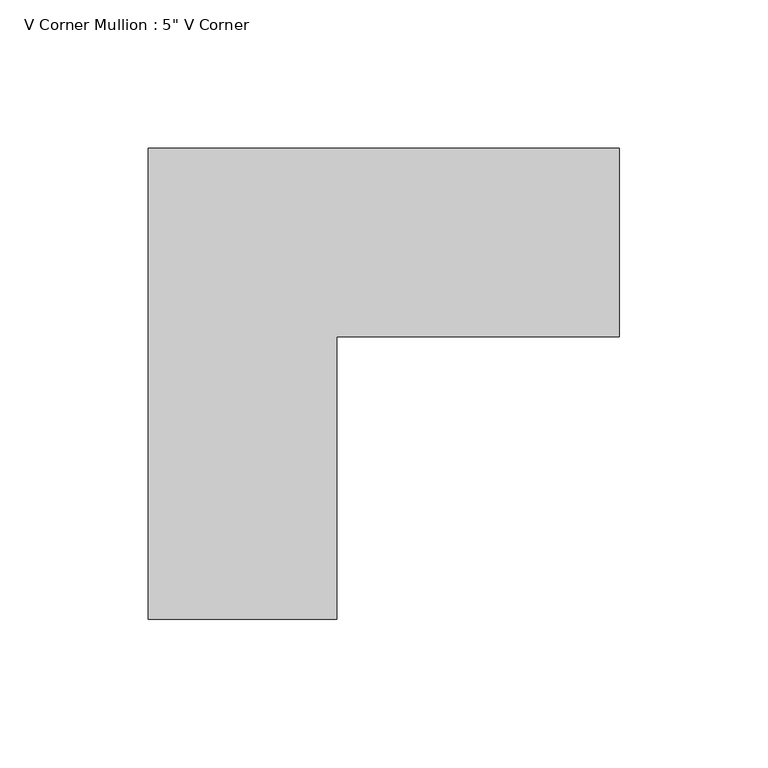
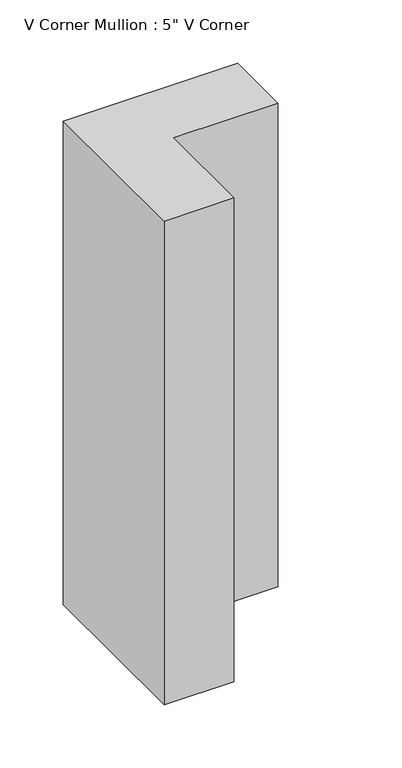
"""IFC4 building model written with IfcOpenShell, lengths in millimetres: member geometry."""

from ifc_helpers import new_model, si_unit, frame, origin, place, context, project, spatial, polyline, outline, extrude, source, transform, mapped, element, save


def member_73de4bef(model_context):
    return source(origin(), model_context, "Body", "SweptSolid", [
        extrude(outline(polyline([(63.5, 31.75), (-31.75, 31.75), (-31.75, -63.5), (-95.25, -63.5), (-95.25, 95.25), (63.5, 95.25), (63.5, 31.75)])), frame((0.0, 0.0, -465.6666667), z_axis=(0.0, 0.0, 1.0), x_axis=(1.0, 0.0, 0.0)), (0.0, 0.0, 1.0), 465.6666667),
    ])


if __name__ == "__main__":
    model = new_model("IFC4")
    model_context = context("Model", 3, world=origin())
    ifc_project = project(units=[si_unit("LENGTHUNIT", "METRE", prefix="MILLI")], contexts=[model_context])
    site = spatial("IfcSite", under=ifc_project)
    building = spatial("IfcBuilding", under=site)
    placement = place(None, origin())
    member_shape = member_73de4bef(model_context)
    element("IfcMember", 1, ObjectType="V Corner Mullion : 5\" V Corner", at=placement, inside=building, context=model_context, shape_type="MappedRepresentation", body=[
        mapped(member_shape, transform((0.0, 0.0, 0.0), x_axis=(1.0, 0.0, 0.0), y_axis=(0.0, 1.0, 0.0), z_axis=(0.0, 0.0, 1.0))),
    ])
    save(model, "model.ifc")

# Revit data of these elements
# Type "V Corner Mullion : 5\" V Corner"
#   built-in parameter 1007355 = 0.416667 (stored number, unit not read)
#   built-in parameter 1007354 = 0.416667 (stored number, unit not read)
#   built-in parameter 1007304 = 0.208333 (stored number, unit not read)
# Element 1 (IfcMember, "V Corner Mullion : 5\" V Corner")
#   Materials on its faces: "Aluminum"
# Materials
#   "Aluminum": class "Metal", colour RGB 244 245 246, transparency 0, Description = "Aluminum 6061", Cost = 0
